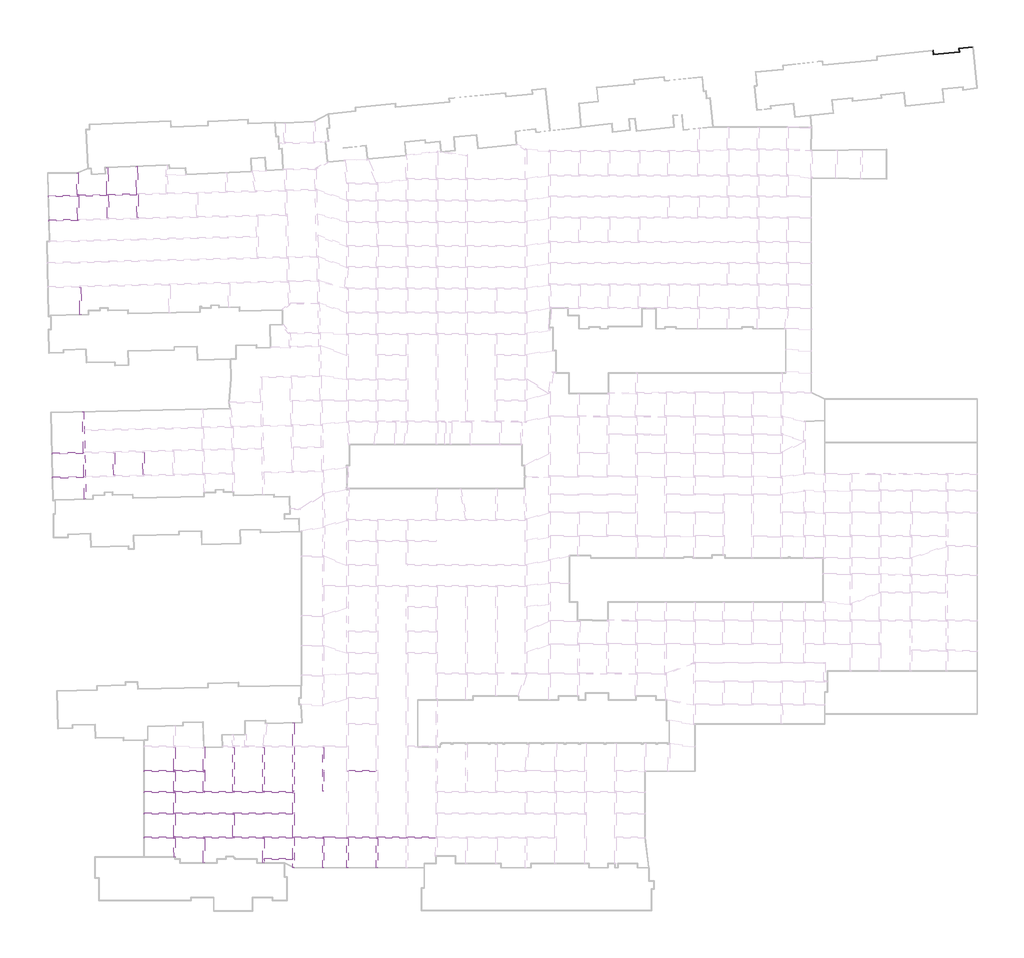
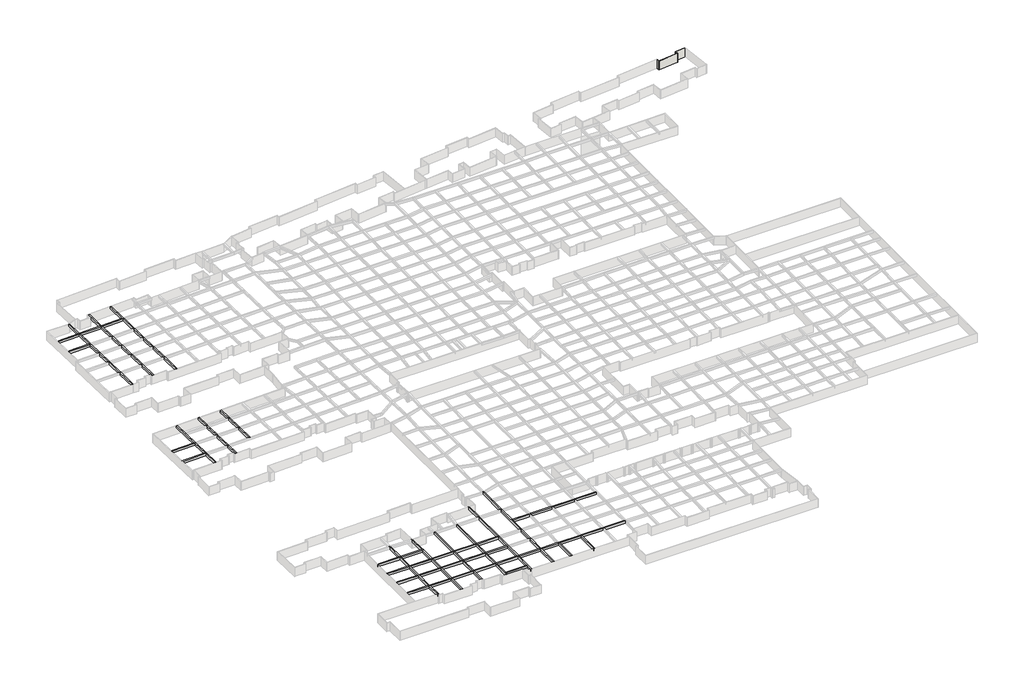
# One storey, part 8 of 20: 42 beams, 4 walls.
"""IFC4 building model written with IfcOpenShell, lengths in millimetres."""

from ifc_helpers import new_model, si_unit, frame, origin, place, context, project, spatial, polyline, outline, extrude, faceted_brep, element, save

model = new_model("IFC4")

# Units and contexts
model_context = context("Model", 3, world=origin())
ifc_project = project(units=[si_unit("LENGTHUNIT", "METRE", prefix="MILLI")], contexts=[model_context])

# Site, building, storey
site = spatial("IfcSite", under=ifc_project)
building = spatial("IfcBuilding", under=site)
storey = spatial("IfcBuildingStorey", under=building, Name="户型图", Elevation=0.0)

# Beams
placement = place(None, origin())
element("IfcBeam", 1, ObjectType="混凝土 - 矩形梁 : KL_beam", at=placement, inside=storey, context=model_context, shape_type="Brep", body=[
    faceted_brep([(-25685.9584576, 180218.1468317, 3300.0), (-25695.523539, 180618.0324519, 3300.0), (-25695.523539, 180618.0324519, 2500.0), (-25685.9584576, 180218.1468317, 2500.0), (-17988.1602694, 180402.2746492, 3300.0), (-17588.2746492, 180411.8397306, 3300.0), (-17597.8397306, 180811.7253508, 3300.0), (-17997.7253508, 180802.1602694, 3300.0), (-17597.8397306, 180811.7253508, 2500.0), (-17997.7253508, 180802.1602694, 2500.0), (-17588.2746492, 180411.8397306, 2500.0), (-17988.1602694, 180402.2746492, 2500.0)], [[[0, 1, 2, 3]], [[1, 0, 4, 5, 6, 7]], [[2, 1, 7, 6, 8, 9]], [[3, 2, 9, 8, 10, 11]], [[0, 3, 11, 10, 5, 4]], [[6, 5, 10, 8]]]),
])
element("IfcBeam", 2, ObjectType="混凝土 - 矩形梁 : KL_beam", at=placement, inside=storey, context=model_context, shape_type="Brep", body=[
    faceted_brep([(-17832.7062646, 173903.2373381, 3300.0), (-17432.8206445, 173912.8024195, 3300.0), (-17442.3866011, 174312.7246305, 3300.0), (-17588.2746492, 180411.8397306, 3300.0), (-17988.1602694, 180402.2746492, 3300.0), (-17842.2713461, 174303.1229582, 3300.0), (-17832.7062646, 173903.2373381, 2500.0), (-17988.1602694, 180402.2746492, 2500.0), (-17842.2713461, 174303.1229582, 2500.0), (-17432.8206445, 173912.8024195, 2500.0), (-17588.2746492, 180411.8397306, 2500.0), (-17442.3866011, 174312.7246305, 2500.0)], [[[0, 1, 2, 3, 4, 5]], [[6, 0, 5, 4, 7, 8]], [[9, 6, 8, 7, 10, 11]], [[1, 9, 11, 10, 3, 2]], [[4, 3, 10, 7]], [[1, 0, 6, 9]]]),
])
element("IfcBeam", 3, ObjectType="混凝土 - 矩形梁 : KL_beam", at=placement, inside=storey, context=model_context, shape_type="SweptSolid", body=[
    extrude(outline(polyline([(-25579.9010779, 173717.9279759), (-25589.4661593, 174117.813596), (-17842.2713461, 174303.1229582), (-17832.7062646, 173903.2373381), (-25579.9010779, 173717.9279759)])), frame((0.0, 0.0, 2500.0), z_axis=(0.0, 0.0, 1.0), x_axis=(1.0, 0.0, 0.0)), (0.0, 0.0, 1.0), 800.0),
])
element("IfcBeam", 4, ObjectType="混凝土 - 矩形梁 : KL_beam", at=placement, inside=storey, context=model_context, shape_type="SweptSolid", body=[
    extrude(outline(polyline([(-17597.8397306, 180811.7253508), (-17997.7253508, 180802.1602694), (-18138.5658972, 186690.2553865), (-17949.102694, 186690.2553865), (-17740.5687803, 186778.7727812), (-17597.8397306, 180811.7253508)])), frame((0.0, 0.0, 2500.0), z_axis=(0.0, 0.0, 1.0), x_axis=(1.0, 0.0, 0.0)), (0.0, 0.0, 1.0), 800.0),
])
element("IfcBeam", 5, ObjectType="混凝土 - 矩形梁 : KL_beam", at=placement, inside=storey, context=model_context, shape_type="SweptSolid", body=[
    extrude(outline(polyline([(-17588.2750768, 180411.8576065), (-17597.8401582, 180811.7432282), (-9999.8837416, 180994.1625895), (-9990.2703339, 180594.278128), (-17588.2750768, 180411.8576065)])), frame((0.0, 0.0, 2500.0), z_axis=(0.0, 0.0, 1.0), x_axis=(1.0, 0.0, 0.0)), (0.0, 0.0, 1.0), 800.0),
])
element("IfcBeam", 6, ObjectType="混凝土 - 矩形梁 : KL_beam", at=placement, inside=storey, context=model_context, shape_type="SweptSolid", body=[
    extrude(outline(polyline([(-9590.3861591, 180603.9034521), (-9599.9995668, 181003.7879151), (-2006.664785, 181187.0229254), (-1996.9546451, 180787.1407967), (-9590.3861591, 180603.9034521)])), frame((0.0, 0.0, 2500.0), z_axis=(0.0, 0.0, 1.0), x_axis=(1.0, 0.0, 0.0)), (0.0, 0.0, 1.0), 800.0),
])
element("IfcBeam", 7, ObjectType="混凝土 - 矩形梁 : KL_beam", at=placement, inside=storey, context=model_context, shape_type="SweptSolid", body=[
    extrude(outline(polyline([(-16823.0159443, 148613.9916157), (-17222.8998075, 148604.3533596), (-17401.6326758, 156019.8431266), (-17001.7470489, 156029.4082082), (-16823.0159443, 148613.9916157)])), frame((0.0, 0.0, 2500.0), z_axis=(0.0, 0.0, 1.0), x_axis=(1.0, 0.0, 0.0)), (0.0, 0.0, 1.0), 800.0),
    extrude(outline(polyline([(-17832.6696806, 173903.2382131), (-17432.7840537, 173912.8032947), (-17306.2945554, 168664.8509217), (-17706.1801823, 168655.2858401), (-17832.6696806, 173903.2382131)])), frame((0.0, 0.0, 2500.0), z_axis=(0.0, 0.0, 1.0), x_axis=(1.0, 0.0, 0.0)), (0.0, 0.0, 1.0), 800.0),
    extrude(outline(polyline([(-17696.541926, 168255.4019703), (-17296.6562991, 168264.9670519), (-17167.7594012, 162917.1335125), (-17567.6433405, 162907.4984183), (-17696.541926, 168255.4019703)])), frame((0.0, 0.0, 2500.0), z_axis=(0.0, 0.0, 1.0), x_axis=(1.0, 0.0, 0.0)), (0.0, 0.0, 1.0), 800.0),
    extrude(outline(polyline([(-17558.0050844, 162507.6145551), (-17158.121145, 162517.2496493), (-17011.3853052, 156429.292078), (-17411.2709321, 156419.7269964), (-17558.0050844, 162507.6145551)])), frame((0.0, 0.0, 2500.0), z_axis=(0.0, 0.0, 1.0), x_axis=(1.0, 0.0, 0.0)), (0.0, 0.0, 1.0), 800.0),
])
element("IfcBeam", 8, ObjectType="混凝土 - 矩形梁 : KL_beam", at=placement, inside=storey, context=model_context, shape_type="Brep", body=[
    faceted_brep([(-8850.0626403, 149809.0093189, 3300.0), (-9249.9471016, 149799.3959113, 3300.0), (-9249.9471016, 149799.3959113, 2500.0), (-8850.0626403, 149809.0093189, 2500.0), (-9004.2027939, 156220.7058147, 3300.0), (-9404.088417, 156211.1407332, 3300.0), (-9404.088417, 156211.1407332, 2500.0), (-9004.2027939, 156220.7058147, 2500.0)], [[[0, 1, 2, 3]], [[1, 0, 4, 5]], [[2, 1, 5, 6]], [[3, 2, 6, 7]], [[0, 3, 7, 4]], [[5, 4, 7, 6]]]),
    faceted_brep([(-10170.4329888, 188088.4205433, 3300.0), (-9770.7457256, 188106.2367096, 3300.0), (-9770.7457256, 188106.2367096, 2500.0), (-10170.4329888, 188088.4205433, 2500.0), (-9443.7780087, 174505.5122009, 3300.0), (-9843.6618727, 174495.8739447, 3300.0), (-9843.6618727, 174495.8739447, 2500.0), (-9443.7780087, 174505.5122009, 2500.0), (-9999.8837416, 180994.1625895, 3300.0), (-9990.2703339, 180594.278128, 3300.0), (-9590.3861591, 180603.9034521, 3300.0), (-9599.9995668, 181003.7879151, 3300.0), (-9999.8837416, 180994.1625895, 2500.0), (-9990.2703339, 180594.278128, 2500.0), (-9599.9995668, 181003.7879151, 2500.0), (-9590.3861591, 180603.9034521, 2500.0)], [[[0, 1, 2, 3]], [[4, 5, 6, 7]], [[1, 0, 8, 9, 5, 4, 10, 11]], [[0, 3, 12, 13, 6, 5, 9, 8]], [[3, 2, 14, 15, 7, 6, 13, 12]], [[2, 1, 11, 10, 4, 7, 15, 14]]]),
    faceted_brep([(-9834.048465, 174095.9894827, 3300.0), (-9434.164601, 174105.6277388, 3300.0), (-9434.164601, 174105.6277388, 2500.0), (-9834.048465, 174095.9894827, 2500.0), (-9307.9651408, 168856.1673089, 3300.0), (-9707.8507639, 168846.6022274, 3300.0), (-9707.8507639, 168846.6022274, 2500.0), (-9307.9651408, 168856.1673089, 2500.0)], [[[0, 1, 2, 3]], [[4, 5, 6, 7]], [[1, 0, 5, 4]], [[0, 3, 6, 5]], [[3, 2, 7, 6]], [[2, 1, 4, 7]]]),
    faceted_brep([(-9698.2373562, 168446.7177632, 3300.0), (-9298.3517331, 168456.2828447, 3300.0), (-9298.3517331, 168456.2828447, 2500.0), (-9698.2373562, 168446.7177632, 2500.0), (-9169.8208105, 163109.841657, 3300.0), (-9569.7047505, 163100.2065627, 3300.0), (-9569.7047505, 163100.2065627, 2500.0), (-9169.8208105, 163109.841657, 2500.0)], [[[0, 1, 2, 3]], [[4, 5, 6, 7]], [[1, 0, 5, 4]], [[0, 3, 6, 5]], [[3, 2, 7, 6]], [[2, 1, 4, 7]]]),
    faceted_brep([(-9560.0913428, 162700.3221009, 3300.0), (-9160.2074028, 162709.9571951, 3300.0), (-9160.2074028, 162709.9571951, 2500.0), (-9560.0913428, 162700.3221009, 2500.0), (-9013.8162016, 156620.5902789, 3300.0), (-9413.7018247, 156611.0251974, 3300.0), (-9413.7018247, 156611.0251974, 2500.0), (-9013.8162016, 156620.5902789, 2500.0)], [[[0, 1, 2, 3]], [[4, 5, 6, 7]], [[1, 0, 5, 4]], [[0, 3, 6, 5]], [[3, 2, 7, 6]], [[2, 1, 4, 7]]]),
])
element("IfcBeam", 9, ObjectType="混凝土 - 矩形梁 : KL_beam", at=placement, inside=storey, context=model_context, shape_type="Brep", body=[
    faceted_brep([(-1224.9412784, 148994.1538412, 3300.0), (-1224.9412784, 148994.1538412, 2500.0), (-825.0591543, 149003.8639809, 2500.0), (-825.0591543, 149003.8639809, 3300.0), (-1404.8339776, 156402.4792466, 3300.0), (-1004.9483311, 156412.0443286, 3300.0), (-1004.9483311, 156412.0443286, 2500.0), (-1404.8339776, 156402.4792466, 2500.0)], [[[0, 1, 2, 3]], [[4, 5, 6, 7]], [[0, 3, 5, 4]], [[3, 2, 6, 5]], [[2, 1, 7, 6]], [[1, 0, 4, 7]]]),
    faceted_brep([(-1783.2084216, 188462.2833149, 3300.0), (-2182.8937132, 188444.4672364, 3300.0), (-2006.664785, 181187.0229254, 3300.0), (-1996.9546451, 180787.1407967, 3300.0), (-1848.8660596, 174688.5696172, 3300.0), (-1448.98219, 174698.2078735, 3300.0), (-1597.0758138, 180796.9865396, 3300.0), (-1606.785957, 181196.8688079, 3300.0), (-1783.2084216, 188462.2833149, 2500.0), (-1448.98219, 174698.2078735, 2500.0), (-1597.0758138, 180796.9865396, 2500.0), (-1606.785957, 181196.8688079, 2500.0), (-2182.8937132, 188444.4672364, 2500.0), (-1848.8660596, 174688.5696172, 2500.0), (-1996.9546451, 180787.1407967, 2500.0), (-2006.664785, 181187.0229254, 2500.0)], [[[0, 1, 2, 3, 4, 5, 6, 7]], [[8, 0, 7, 6, 5, 9, 10, 11]], [[12, 8, 11, 10, 9, 13, 14, 15]], [[1, 12, 15, 14, 13, 4, 3, 2]], [[1, 0, 8, 12]], [[5, 4, 13, 9]]]),
    faceted_brep([(-1839.1559197, 174288.6874866, 3300.0), (-1439.2720501, 174298.3257429, 3300.0), (-1439.2720501, 174298.3257429, 2500.0), (-1839.1559197, 174288.6874866, 2500.0), (-1711.65286, 169037.8676298, 3300.0), (-1311.7672135, 169047.4327119, 3300.0), (-1311.7672135, 169047.4327119, 2500.0), (-1711.65286, 169037.8676298, 2500.0)], [[[0, 1, 2, 3]], [[1, 0, 4, 5]], [[2, 1, 5, 6]], [[3, 2, 6, 7]], [[0, 3, 7, 4]], [[5, 4, 7, 6]]]),
    faceted_brep([(-1701.9427196, 168637.9854794, 3300.0), (-1302.0570732, 168647.5505615, 3300.0), (-1302.0570732, 168647.5505615, 2500.0), (-1701.9427196, 168637.9854794, 2500.0), (-1572.1507865, 163292.9054397, 3300.0), (-1172.2668401, 163302.5405341, 3300.0), (-1172.2668401, 163302.5405341, 2500.0), (-1572.1507865, 163292.9054397, 2500.0)], [[[0, 1, 2, 3]], [[1, 0, 4, 5]], [[2, 1, 5, 6]], [[3, 2, 6, 7]], [[0, 3, 7, 4]], [[5, 4, 7, 6]]]),
    faceted_brep([(-1562.4406466, 162893.0233086, 3300.0), (-1162.5567002, 162902.658403, 3300.0), (-1162.5567002, 162902.658403, 2500.0), (-1562.4406466, 162893.0233086, 2500.0), (-1414.5441179, 156802.361397, 3300.0), (-1014.6584715, 156811.926479, 3300.0), (-1014.6584715, 156811.926479, 2500.0), (-1414.5441179, 156802.361397, 2500.0)], [[[0, 1, 2, 3]], [[1, 0, 4, 5]], [[2, 1, 5, 6]], [[3, 2, 6, 7]], [[0, 3, 7, 4]], [[5, 4, 7, 6]]]),
])
element("IfcBeam", 10, ObjectType="混凝土 - 矩形梁 : KL_beam", at=placement, inside=storey, context=model_context, shape_type="SweptSolid", body=[
    extrude(outline(polyline([(54450.0, 26240.0), (54450.0, 25840.0), (48350.0, 25840.0), (48350.0, 26240.0), (54450.0, 26240.0)])), frame((0.0, 0.0, 2500.0), z_axis=(0.0, 0.0, 1.0), x_axis=(1.0, 0.0, 0.0)), (0.0, 0.0, 1.0), 800.0),
    extrude(outline(polyline([(78450.0, 26240.0), (78450.0, 25840.0), (70850.0, 25840.0), (70850.0, 26240.0), (78450.0, 26240.0)])), frame((0.0, 0.0, 2500.0), z_axis=(0.0, 0.0, 1.0), x_axis=(1.0, 0.0, 0.0)), (0.0, 0.0, 1.0), 800.0),
    extrude(outline(polyline([(70450.0, 26240.0), (70450.0, 25840.0), (62850.0, 25840.0), (62850.0, 26240.0), (70450.0, 26240.0)])), frame((0.0, 0.0, 2500.0), z_axis=(0.0, 0.0, 1.0), x_axis=(1.0, 0.0, 0.0)), (0.0, 0.0, 1.0), 800.0),
    extrude(outline(polyline([(62450.0, 26240.0), (62450.0, 25840.0), (54850.0, 25840.0), (54850.0, 26240.0), (62450.0, 26240.0)])), frame((0.0, 0.0, 2500.0), z_axis=(0.0, 0.0, 1.0), x_axis=(1.0, 0.0, 0.0)), (0.0, 0.0, 1.0), 800.0),
])
element("IfcBeam", 11, ObjectType="混凝土 - 矩形梁 : KL_beam", at=placement, inside=storey, context=model_context, shape_type="Brep", body=[
    faceted_brep([(78450.0, 7940.0, 3300.0), (78450.0, 8340.0, 3300.0), (70850.0, 8340.0, 3300.0), (70450.0, 8340.0, 3300.0), (62850.0, 8340.0, 3300.0), (62450.0, 8340.0, 3300.0), (54850.0, 8340.0, 3300.0), (54450.0, 8340.0, 3300.0), (48350.0, 8340.0, 3300.0), (47950.0, 8340.0, 3300.0), (40351.7306283, 8340.0, 3300.0), (40351.7306283, 7940.0, 3300.0), (47950.0, 7940.0, 3300.0), (48350.0, 7940.0, 3300.0), (54450.0, 7940.0, 3300.0), (54850.0, 7940.0, 3300.0), (62450.0, 7940.0, 3300.0), (62850.0, 7940.0, 3300.0), (70450.0, 7940.0, 3300.0), (70850.0, 7940.0, 3300.0), (78440.7384461, 7940.0, 3300.0), (78450.0, 8340.0, 2500.0), (70850.0, 8340.0, 2500.0), (70450.0, 8340.0, 2500.0), (62850.0, 8340.0, 2500.0), (62450.0, 8340.0, 2500.0), (54850.0, 8340.0, 2500.0), (54450.0, 8340.0, 2500.0), (48350.0, 8340.0, 2500.0), (47950.0, 8340.0, 2500.0), (40351.7306283, 8340.0, 2500.0), (78450.0, 7940.0, 2500.0), (78440.7384461, 7940.0, 2500.0), (70850.0, 7940.0, 2500.0), (70450.0, 7940.0, 2500.0), (62850.0, 7940.0, 2500.0), (62450.0, 7940.0, 2500.0), (54850.0, 7940.0, 2500.0), (54450.0, 7940.0, 2500.0), (48350.0, 7940.0, 2500.0), (47950.0, 7940.0, 2500.0), (40351.7306283, 7940.0, 2500.0)], [[[0, 1, 2, 3, 4, 5, 6, 7, 8, 9, 10, 11, 12, 13, 14, 15, 16, 17, 18, 19, 20]], [[1, 21, 22, 23, 24, 25, 26, 27, 28, 29, 30, 10, 9, 8, 7, 6, 5, 4, 3, 2]], [[21, 31, 32, 33, 34, 35, 36, 37, 38, 39, 40, 41, 30, 29, 28, 27, 26, 25, 24, 23, 22]], [[31, 0, 20, 19, 18, 17, 16, 15, 14, 13, 12, 11, 41, 40, 39, 38, 37, 36, 35, 34, 33, 32]], [[1, 0, 31, 21]], [[11, 10, 30, 41]]]),
])
element("IfcBeam", 12, ObjectType="混凝土 - 矩形梁 : KL_beam", at=placement, inside=storey, context=model_context, shape_type="SweptSolid", body=[
    extrude(outline(polyline([(23892.5739519, 32340.0), (24292.5739519, 32340.0), (24292.5739519, 20540.0), (23892.5739519, 20540.0), (23892.5739519, 32340.0)])), frame((0.0, 0.0, 2500.0), z_axis=(0.0, 0.0, 1.0), x_axis=(1.0, 0.0, 0.0)), (0.0, 0.0, 1.0), 800.0),
])
element("IfcBeam", 13, ObjectType="混凝土 - 矩形梁 : KL_beam", at=placement, inside=storey, context=model_context, shape_type="SweptSolid", body=[
    extrude(outline(polyline([(31950.0, 32340.0), (32350.0, 32340.0), (32350.0, 20540.0), (31950.0, 20540.0), (31950.0, 32340.0)])), frame((0.0, 0.0, 2500.0), z_axis=(0.0, 0.0, 1.0), x_axis=(1.0, 0.0, 0.0)), (0.0, 0.0, 1.0), 800.0),
])
element("IfcBeam", 14, ObjectType="混凝土 - 矩形梁 : KL_beam", at=placement, inside=storey, context=model_context, shape_type="Brep", body=[
    faceted_brep([(40351.7306283, 38946.111756, 3300.0), (40351.7306283, 38946.111756, 2500.0), (39951.7306283, 38946.111756, 2500.0), (39951.7306283, 38946.111756, 3300.0), (39951.7306283, 32740.0, 3300.0), (39951.7306283, 32340.0, 3300.0), (39951.7306283, 20540.0, 3300.0), (40351.7306283, 20540.0, 3300.0), (40351.7306283, 32340.0, 3300.0), (40351.7306283, 32740.0, 3300.0), (39951.7306283, 32740.0, 2500.0), (39951.7306283, 32340.0, 2500.0), (39951.7306283, 20540.0, 2500.0), (40351.7306283, 32740.0, 2500.0), (40351.7306283, 32340.0, 2500.0), (40351.7306283, 20540.0, 2500.0)], [[[0, 1, 2, 3]], [[0, 3, 4, 5, 6, 7, 8, 9]], [[3, 2, 10, 11, 12, 6, 5, 4]], [[2, 1, 13, 14, 15, 12, 11, 10]], [[1, 0, 9, 8, 7, 15, 14, 13]], [[7, 6, 12, 15]]]),
])
element("IfcBeam", 15, ObjectType="混凝土 - 矩形梁 : KL_beam", at=placement, inside=storey, context=model_context, shape_type="Brep", body=[
    faceted_brep([(7945.5604023, 20540.0, 3300.0), (7945.5604023, 20140.0, 3300.0), (8345.5604023, 20140.0, 3300.0), (15956.0, 20140.0, 3300.0), (16356.0, 20140.0, 3300.0), (23892.5739519, 20140.0, 3300.0), (24292.5739519, 20140.0, 3300.0), (31950.0, 20140.0, 3300.0), (32350.0, 20140.0, 3300.0), (39951.7306283, 20140.0, 3300.0), (39951.7306283, 20540.0, 3300.0), (32350.0, 20540.0, 3300.0), (31950.0, 20540.0, 3300.0), (24292.5739519, 20540.0, 3300.0), (23892.5739519, 20540.0, 3300.0), (16356.0, 20540.0, 3300.0), (15956.0, 20540.0, 3300.0), (8345.5604023, 20540.0, 3300.0), (7945.5604023, 20540.0, 2500.0), (39951.7306283, 20540.0, 2500.0), (32350.0, 20540.0, 2500.0), (31950.0, 20540.0, 2500.0), (24292.5739519, 20540.0, 2500.0), (23892.5739519, 20540.0, 2500.0), (16356.0, 20540.0, 2500.0), (15956.0, 20540.0, 2500.0), (8345.5604023, 20540.0, 2500.0), (7945.5604023, 20140.0, 2500.0), (39951.7306283, 20140.0, 2500.0), (32350.0, 20140.0, 2500.0), (31950.0, 20140.0, 2500.0), (24292.5739519, 20140.0, 2500.0), (23892.5739519, 20140.0, 2500.0), (16356.0, 20140.0, 2500.0), (15956.0, 20140.0, 2500.0), (8345.5604023, 20140.0, 2500.0)], [[[0, 1, 2, 3, 4, 5, 6, 7, 8, 9, 10, 11, 12, 13, 14, 15, 16, 17]], [[18, 0, 17, 16, 15, 14, 13, 12, 11, 10, 19, 20, 21, 22, 23, 24, 25, 26]], [[27, 18, 26, 25, 24, 23, 22, 21, 20, 19, 28, 29, 30, 31, 32, 33, 34, 35]], [[1, 27, 35, 34, 33, 32, 31, 30, 29, 28, 9, 8, 7, 6, 5, 4, 3, 2]], [[10, 9, 28, 19]], [[1, 0, 18, 27]]]),
])
element("IfcBeam", 16, ObjectType="混凝土 - 矩形梁 : KL_beam", at=placement, inside=storey, context=model_context, shape_type="Brep", body=[
    faceted_brep([(39951.7306283, 14440.0, 3300.0), (39951.7306283, 14840.0, 3300.0), (32350.0, 14840.0, 3300.0), (31950.0, 14840.0, 3300.0), (24292.5739519, 14840.0, 3300.0), (23892.5739519, 14840.0, 3300.0), (16356.0, 14840.0, 3300.0), (15956.0, 14840.0, 3300.0), (8345.5604023, 14840.0, 3300.0), (8345.5604023, 14440.0, 3300.0), (15956.0, 14440.0, 3300.0), (16356.0, 14440.0, 3300.0), (23892.5739519, 14440.0, 3300.0), (24292.5739519, 14440.0, 3300.0), (31950.0, 14440.0, 3300.0), (32350.0, 14440.0, 3300.0), (39951.7306283, 14440.0, 2500.0), (8345.5604023, 14440.0, 2500.0), (15956.0, 14440.0, 2500.0), (16356.0, 14440.0, 2500.0), (23892.5739519, 14440.0, 2500.0), (24292.5739519, 14440.0, 2500.0), (31950.0, 14440.0, 2500.0), (32350.0, 14440.0, 2500.0), (39951.7306283, 14840.0, 2500.0), (8345.5604023, 14840.0, 2500.0), (15956.0, 14840.0, 2500.0), (16356.0, 14840.0, 2500.0), (23892.5739519, 14840.0, 2500.0), (24292.5739519, 14840.0, 2500.0), (31950.0, 14840.0, 2500.0), (32350.0, 14840.0, 2500.0)], [[[0, 1, 2, 3, 4, 5, 6, 7, 8, 9, 10, 11, 12, 13, 14, 15]], [[16, 0, 15, 14, 13, 12, 11, 10, 9, 17, 18, 19, 20, 21, 22, 23]], [[24, 16, 23, 22, 21, 20, 19, 18, 17, 25, 26, 27, 28, 29, 30, 31]], [[1, 24, 31, 30, 29, 28, 27, 26, 25, 8, 7, 6, 5, 4, 3, 2]], [[1, 0, 16, 24]], [[9, 8, 25, 17]]]),
])
element("IfcBeam", 17, ObjectType="混凝土 - 矩形梁 : KL_beam", at=placement, inside=storey, context=model_context, shape_type="Brep", body=[
    faceted_brep([(7945.5604023, 8340.0, 3300.0), (7945.5604023, 7940.0, 3300.0), (7951.9679234, 7940.0, 3300.0), (8352.1799995, 7940.0, 3300.0), (15956.0, 7940.0, 3300.0), (16356.0, 7940.0, 3300.0), (23892.5739519, 7940.0, 3300.0), (24292.5739519, 7940.0, 3300.0), (31950.0, 7940.0, 3300.0), (32350.0, 7940.0, 3300.0), (39951.7306283, 7940.0, 3300.0), (39951.7306283, 8340.0, 3300.0), (32350.0, 8340.0, 3300.0), (31950.0, 8340.0, 3300.0), (24292.5739519, 8340.0, 3300.0), (23892.5739519, 8340.0, 3300.0), (16356.0, 8340.0, 3300.0), (15956.0, 8340.0, 3300.0), (8345.5604023, 8340.0, 3300.0), (7945.5604023, 8340.0, 2500.0), (39951.7306283, 8340.0, 2500.0), (32350.0, 8340.0, 2500.0), (31950.0, 8340.0, 2500.0), (24292.5739519, 8340.0, 2500.0), (23892.5739519, 8340.0, 2500.0), (16356.0, 8340.0, 2500.0), (15956.0, 8340.0, 2500.0), (8345.5604023, 8340.0, 2500.0), (7945.5604023, 7940.0, 2500.0), (39951.7306283, 7940.0, 2500.0), (32350.0, 7940.0, 2500.0), (31950.0, 7940.0, 2500.0), (24292.5739519, 7940.0, 2500.0), (23892.5739519, 7940.0, 2500.0), (16356.0, 7940.0, 2500.0), (15956.0, 7940.0, 2500.0), (8352.1799995, 7940.0, 2500.0), (7951.9679234, 7940.0, 2500.0)], [[[0, 1, 2, 3, 4, 5, 6, 7, 8, 9, 10, 11, 12, 13, 14, 15, 16, 17, 18]], [[19, 0, 18, 17, 16, 15, 14, 13, 12, 11, 20, 21, 22, 23, 24, 25, 26, 27]], [[28, 19, 27, 26, 25, 24, 23, 22, 21, 20, 29, 30, 31, 32, 33, 34, 35, 36, 37]], [[1, 28, 37, 36, 35, 34, 33, 32, 31, 30, 29, 10, 9, 8, 7, 6, 5, 4, 3, 2]], [[11, 10, 29, 20]], [[1, 0, 19, 28]]]),
])
element("IfcBeam", 18, ObjectType="混凝土 - 矩形梁 : KL_beam", at=placement, inside=storey, context=model_context, shape_type="SweptSolid", body=[
    extrude(outline(polyline([(16356.0, 1311.0), (15956.0, 1311.0), (15956.0, 7940.0), (16356.0, 7940.0), (16356.0, 1311.0)])), frame((0.0, 0.0, 2500.0), z_axis=(0.0, 0.0, 1.0), x_axis=(1.0, 0.0, 0.0)), (0.0, 0.0, 1.0), 800.0),
    extrude(outline(polyline([(15956.0, 20140.0), (16356.0, 20140.0), (16356.0, 14840.0), (15956.0, 14840.0), (15956.0, 20140.0)])), frame((0.0, 0.0, 2500.0), z_axis=(0.0, 0.0, 1.0), x_axis=(1.0, 0.0, 0.0)), (0.0, 0.0, 1.0), 800.0),
    extrude(outline(polyline([(15956.0, 14440.0), (16356.0, 14440.0), (16356.0, 8340.0), (15956.0, 8340.0), (15956.0, 14440.0)])), frame((0.0, 0.0, 2500.0), z_axis=(0.0, 0.0, 1.0), x_axis=(1.0, 0.0, 0.0)), (0.0, 0.0, 1.0), 800.0),
])
element("IfcBeam", 19, ObjectType="混凝土 - 矩形梁 : KL_beam", at=placement, inside=storey, context=model_context, shape_type="SweptSolid", body=[
    extrude(outline(polyline([(24292.5739519, 3040.0), (23892.5739519, 3040.0), (23892.5739519, 7940.0), (24292.5739519, 7940.0), (24292.5739519, 3040.0)])), frame((0.0, 0.0, 2500.0), z_axis=(0.0, 0.0, 1.0), x_axis=(1.0, 0.0, 0.0)), (0.0, 0.0, 1.0), 800.0),
    extrude(outline(polyline([(23892.5739519, 20140.0), (24292.5739519, 20140.0), (24292.5739519, 14840.0), (23892.5739519, 14840.0), (23892.5739519, 20140.0)])), frame((0.0, 0.0, 2500.0), z_axis=(0.0, 0.0, 1.0), x_axis=(1.0, 0.0, 0.0)), (0.0, 0.0, 1.0), 800.0),
    extrude(outline(polyline([(23892.5739519, 14440.0), (24292.5739519, 14440.0), (24292.5739519, 8340.0), (23892.5739519, 8340.0), (23892.5739519, 14440.0)])), frame((0.0, 0.0, 2500.0), z_axis=(0.0, 0.0, 1.0), x_axis=(1.0, 0.0, 0.0)), (0.0, 0.0, 1.0), 800.0),
])
element("IfcBeam", 20, ObjectType="混凝土 - 矩形梁 : KL_beam", at=placement, inside=storey, context=model_context, shape_type="Brep", body=[
    faceted_brep([(32350.0, 1311.0, 3300.0), (31950.0, 1311.0, 3300.0), (31950.0, 1311.0, 2500.0), (32350.0, 1311.0, 2500.0), (32350.0, 2170.0, 3300.0), (32350.0, 2570.0, 3300.0), (32350.0, 7940.0, 3300.0), (31950.0, 7940.0, 3300.0), (31950.0, 7940.0, 2500.0), (32350.0, 7940.0, 2500.0), (32350.0, 2570.0, 2500.0), (32350.0, 2170.0, 2500.0)], [[[0, 1, 2, 3]], [[1, 0, 4, 5, 6, 7]], [[2, 1, 7, 8]], [[3, 2, 8, 9, 10, 11]], [[0, 3, 11, 10, 9, 6, 5, 4]], [[7, 6, 9, 8]]]),
    faceted_brep([(31950.0, 20140.0, 3300.0), (32350.0, 20140.0, 3300.0), (32350.0, 20140.0, 2500.0), (31950.0, 20140.0, 2500.0), (32350.0, 14840.0, 3300.0), (31950.0, 14840.0, 3300.0), (31950.0, 14840.0, 2500.0), (32350.0, 14840.0, 2500.0)], [[[0, 1, 2, 3]], [[4, 5, 6, 7]], [[1, 0, 5, 4]], [[0, 3, 6, 5]], [[3, 2, 7, 6]], [[2, 1, 4, 7]]]),
    faceted_brep([(31950.0, 14440.0, 3300.0), (32350.0, 14440.0, 3300.0), (32350.0, 14440.0, 2500.0), (31950.0, 14440.0, 2500.0), (32350.0, 8340.0, 3300.0), (31950.0, 8340.0, 3300.0), (31950.0, 8340.0, 2500.0), (32350.0, 8340.0, 2500.0)], [[[0, 1, 2, 3]], [[4, 5, 6, 7]], [[1, 0, 5, 4]], [[0, 3, 6, 5]], [[3, 2, 7, 6]], [[2, 1, 4, 7]]]),
])
element("IfcBeam", 21, ObjectType="混凝土 - 矩形梁 : KL_beam", at=placement, inside=storey, context=model_context, shape_type="Brep", body=[
    faceted_brep([(40351.7306283, -3.2601879, 3300.0), (39951.7306283, -3.2601879, 3300.0), (39951.7306283, -3.2601879, 2500.0), (40351.7306283, -3.2601879, 2500.0), (40351.7306283, 7940.0, 3300.0), (40351.7306283, 8340.0, 3300.0), (40351.7306283, 14440.0, 3300.0), (40351.7306283, 14840.0, 3300.0), (40351.7306283, 20140.0, 3300.0), (39951.7306283, 20140.0, 3300.0), (39951.7306283, 14840.0, 3300.0), (39951.7306283, 14440.0, 3300.0), (39951.7306283, 8340.0, 3300.0), (39951.7306283, 7940.0, 3300.0), (39951.7306283, 2570.0, 3300.0), (39951.7306283, 2170.0, 3300.0), (39951.7306283, 20140.0, 2500.0), (39951.7306283, 14840.0, 2500.0), (39951.7306283, 14440.0, 2500.0), (39951.7306283, 8340.0, 2500.0), (39951.7306283, 7940.0, 2500.0), (39951.7306283, 2570.0, 2500.0), (39951.7306283, 2170.0, 2500.0), (40351.7306283, 20140.0, 2500.0), (40351.7306283, 14840.0, 2500.0), (40351.7306283, 14440.0, 2500.0), (40351.7306283, 8340.0, 2500.0), (40351.7306283, 7940.0, 2500.0)], [[[0, 1, 2, 3]], [[1, 0, 4, 5, 6, 7, 8, 9, 10, 11, 12, 13, 14, 15]], [[2, 1, 15, 14, 13, 12, 11, 10, 9, 16, 17, 18, 19, 20, 21, 22]], [[3, 2, 22, 21, 20, 19, 18, 17, 16, 23, 24, 25, 26, 27]], [[0, 3, 27, 26, 25, 24, 23, 8, 7, 6, 5, 4]], [[9, 8, 23, 16]]]),
])
element("IfcBeam", 22, ObjectType="混凝土 - 矩形梁 : KL_beam", at=placement, inside=storey, context=model_context, shape_type="SweptSolid", body=[
    extrude(outline(polyline([(32350.0, 2170.0), (32350.0, 2570.0), (39951.7306283, 2570.0), (39951.7306283, 2170.0), (32350.0, 2170.0)])), frame((0.0, 0.0, 2500.0), z_axis=(0.0, 0.0, 1.0), x_axis=(1.0, 0.0, 0.0)), (0.0, 0.0, 1.0), 800.0),
])
element("IfcBeam", 23, ObjectType="混凝土 - 矩形梁 : KL_beam", at=placement, inside=storey, context=model_context, shape_type="Brep", body=[
    faceted_brep([(47950.0, 8340.0, 3300.0), (48350.0, 8340.0, 3300.0), (48350.0, 14440.0, 3300.0), (47950.0, 14440.0, 3300.0), (47950.0, 8340.0, 2500.0), (47950.0, 14440.0, 2500.0), (48350.0, 8340.0, 2500.0), (48350.0, 14440.0, 2500.0)], [[[0, 1, 2, 3]], [[4, 0, 3, 5]], [[6, 4, 5, 7]], [[1, 6, 7, 2]], [[1, 0, 4, 6]], [[3, 2, 7, 5]]]),
    faceted_brep([(48350.0, 14840.0, 3300.0), (47950.0, 14840.0, 3300.0), (47950.0, 14840.0, 2500.0), (48350.0, 14840.0, 2500.0), (48350.0, 20140.0, 3300.0), (47950.0, 20140.0, 3300.0), (47950.0, 20140.0, 2500.0), (48350.0, 20140.0, 2500.0)], [[[0, 1, 2, 3]], [[1, 0, 4, 5]], [[2, 1, 5, 6]], [[3, 2, 6, 7]], [[0, 3, 7, 4]], [[5, 4, 7, 6]]]),
    faceted_brep([(48350.0, 20540.0, 3300.0), (47950.0, 20540.0, 3300.0), (47950.0, 20540.0, 2500.0), (48350.0, 20540.0, 2500.0), (48350.0, 25840.0, 3300.0), (48350.0, 26240.0, 3300.0), (48350.0, 32340.0, 3300.0), (47950.0, 32340.0, 3300.0), (47950.0, 32340.0, 2500.0), (48350.0, 32340.0, 2500.0), (48350.0, 26240.0, 2500.0), (48350.0, 25840.0, 2500.0)], [[[0, 1, 2, 3]], [[1, 0, 4, 5, 6, 7]], [[2, 1, 7, 8]], [[3, 2, 8, 9, 10, 11]], [[0, 3, 11, 10, 9, 6, 5, 4]], [[7, 6, 9, 8]]]),
    faceted_brep([(48350.0, 32740.0, 3300.0), (47950.0, 32740.0, 3300.0), (47950.0, 32740.0, 2500.0), (48350.0, 32740.0, 2500.0), (48350.0, 43852.7641216, 3300.0), (47950.0, 43867.507495, 3300.0), (47950.0, 43467.2358784, 3300.0), (48350.0, 38390.0, 3300.0), (48350.0, 38790.0, 3300.0), (48350.0, 43510.0922713, 3300.0), (47950.0, 43867.507495, 2500.0), (47950.0, 43467.2358784, 2500.0), (48350.0, 43852.7641216, 2500.0), (48350.0, 43510.0922713, 2500.0), (48350.0, 38790.0, 2500.0), (48350.0, 38390.0, 2500.0)], [[[0, 1, 2, 3]], [[4, 5, 6, 1, 0, 7, 8, 9]], [[5, 10, 11, 2, 1, 6]], [[10, 12, 13, 14, 15, 3, 2, 11]], [[12, 4, 9, 8, 7, 0, 3, 15, 14, 13]], [[5, 4, 12, 10]]]),
])
element("IfcBeam", 24, ObjectType="混凝土 - 矩形梁 : KL_beam", at=placement, inside=storey, context=model_context, shape_type="Brep", body=[
    faceted_brep([(16346.5394526, 25840.0, 3300.0), (16346.5394526, 26240.0, 3300.0), (15946.4785214, 26240.0, 3300.0), (8345.5604023, 26240.0, 3300.0), (7945.5604023, 26240.0, 3300.0), (7945.5604023, 25840.0, 3300.0), (8345.5604023, 25840.0, 3300.0), (15956.0, 25840.0, 3300.0), (16346.5394526, 25840.0, 2500.0), (7945.5604023, 25840.0, 2500.0), (8345.5604023, 25840.0, 2500.0), (15956.0, 25840.0, 2500.0), (16346.5394526, 26240.0, 2500.0), (7945.5604023, 26240.0, 2500.0), (8345.5604023, 26240.0, 2500.0), (15946.4785214, 26240.0, 2500.0)], [[[0, 1, 2, 3, 4, 5, 6, 7]], [[8, 0, 7, 6, 5, 9, 10, 11]], [[12, 8, 11, 10, 9, 13, 14, 15]], [[1, 12, 15, 14, 13, 4, 3, 2]], [[1, 0, 8, 12]], [[5, 4, 13, 9]]]),
])
element("IfcBeam", 25, ObjectType="混凝土 - 矩形梁 : KL_beam", at=placement, inside=storey, context=model_context, shape_type="Brep", body=[
    faceted_brep([(16237.4051317, 32492.3010599, 3300.0), (15837.1001969, 32506.2800163, 3300.0), (15844.0907397, 32105.7920834, 3300.0), (15946.4785214, 26240.0, 3300.0), (16346.5394526, 26240.0, 3300.0), (16353.5214786, 25840.0, 3300.0), (16353.5214786, 25840.0, 2500.0), (16350.0304656, 26040.0, 2500.0), (16346.5394526, 26240.0, 2500.0), (16237.4051317, 32492.3010599, 2500.0), (16350.0304656, 26040.0, 3300.0), (15837.1001969, 32506.2800163, 2500.0), (15946.4785214, 26240.0, 2500.0), (15844.0907397, 32105.7920834, 2500.0), (16346.5394526, 25840.0, 3300.0), (16346.5394526, 25840.0, 2500.0)], [[[0, 1, 2, 3, 4]], [[5, 6, 7, 8, 9, 0, 4, 10]], [[11, 9, 8, 12, 13]], [[1, 11, 13, 12, 3, 2]], [[6, 5, 14, 15]], [[8, 4, 3, 12]], [[4, 8, 15, 14]], [[14, 5, 10, 4]], [[8, 7, 6, 15]], [[1, 0, 9, 11]]]),
])
element("IfcBeam", 26, ObjectType="混凝土 - 矩形梁 : KL_beam", at=placement, inside=storey, context=model_context, shape_type="Brep", body=[
    faceted_brep([(7945.5604023, 26240.0, 3300.0), (8345.5604023, 26240.0, 3300.0), (8345.5604023, 32367.6465329, 3300.0), (7945.5604023, 32381.6148407, 3300.0), (7945.5604023, 32374.7525956, 3300.0), (7945.5604023, 32781.8586584, 3300.0), (7945.5604023, 32781.8586584, 2500.0), (7945.5604023, 32774.7525956, 2500.0), (7945.5604023, 32381.6148407, 2500.0), (7945.5604023, 32374.7525956, 2500.0), (7945.5604023, 26240.0, 2500.0), (7945.5604023, 32774.7525956, 3300.0), (8345.5604023, 26240.0, 2500.0), (8345.5604023, 32367.6465329, 2500.0), (7959.5202009, 32781.3711715, 3300.0), (7959.5202009, 32781.3711715, 2500.0)], [[[0, 1, 2, 3, 4]], [[5, 6, 7, 8, 9, 10, 0, 4, 3, 11]], [[12, 10, 9, 8, 13]], [[1, 12, 13, 2]], [[6, 5, 14, 15]], [[1, 0, 10, 12]], [[8, 3, 2, 13]], [[3, 8, 15, 14]], [[14, 5, 11, 3]], [[6, 15, 8, 7]]]),
])
element("IfcBeam", 27, ObjectType="混凝土 - 矩形梁 : KL_beam", at=placement, inside=storey, context=model_context, shape_type="SweptSolid", body=[
    extrude(outline(polyline([(8345.5604023, 20540.0), (7945.5604023, 20540.0), (7945.5604023, 25840.0), (8345.5604023, 25840.0), (8345.5604023, 20540.0)])), frame((0.0, 0.0, 2500.0), z_axis=(0.0, 0.0, 1.0), x_axis=(1.0, 0.0, 0.0)), (0.0, 0.0, 1.0), 800.0),
])
element("IfcBeam", 28, ObjectType="混凝土 - 矩形梁 : KL_beam", at=placement, inside=storey, context=model_context, shape_type="Brep", body=[
    faceted_brep([(16356.0, 26040.0, 3300.0), (16356.0, 26040.0, 2500.0), (16350.0304656, 26040.0, 2500.0), (16350.0304656, 26040.0, 3300.0), (16356.0, 20540.0, 3300.0), (16353.5214786, 25840.0, 3300.0), (16346.5394526, 25840.0, 3300.0), (15956.0, 25840.0, 3300.0), (15956.0, 20540.0, 3300.0), (16356.0, 20540.0, 2500.0), (15956.0, 20540.0, 2500.0), (15956.0, 25840.0, 2500.0), (16346.5394526, 25840.0, 2500.0), (16353.5214786, 25840.0, 2500.0)], [[[0, 1, 2, 3]], [[4, 0, 3, 5, 6, 7, 8]], [[1, 0, 4, 9]], [[1, 9, 10, 11, 12, 13, 2]], [[10, 8, 7, 11]], [[4, 8, 10, 9]], [[5, 13, 12, 11, 7, 6]], [[13, 5, 3, 2]]]),
])
element("IfcBeam", 29, ObjectType="混凝土 - 矩形梁 : KL_beam", at=placement, inside=storey, context=model_context, shape_type="Brep", body=[
    faceted_brep([(8345.5604023, 20140.0, 3300.0), (7945.5604023, 20140.0, 3300.0), (7945.5604023, 14840.0, 3300.0), (7945.5604023, 14440.0, 3300.0), (7945.5604023, 8340.0, 3300.0), (8345.5604023, 8340.0, 3300.0), (8345.5604023, 14440.0, 3300.0), (8345.5604023, 14840.0, 3300.0), (7945.5604023, 20140.0, 2500.0), (7945.5604023, 14840.0, 2500.0), (7945.5604023, 14440.0, 2500.0), (7945.5604023, 8340.0, 2500.0), (8345.5604023, 20140.0, 2500.0), (8345.5604023, 14840.0, 2500.0), (8345.5604023, 14440.0, 2500.0), (8345.5604023, 8340.0, 2500.0)], [[[0, 1, 2, 3, 4, 5, 6, 7]], [[1, 8, 9, 10, 11, 4, 3, 2]], [[8, 12, 13, 14, 15, 11, 10, 9]], [[12, 0, 7, 6, 5, 15, 14, 13]], [[1, 0, 12, 8]], [[5, 4, 11, 15]]]),
])
element("IfcBeam", 30, ObjectType="混凝土 - 矩形梁 : KL_beam", at=placement, inside=storey, context=model_context, shape_type="SweptSolid", body=[
    extrude(outline(polyline([(20.4770061, 7940.0), (20.4770061, 8340.0), (7945.5604023, 8340.0), (7945.5604023, 7940.0), (20.4770061, 7940.0)])), frame((0.0, 0.0, 2500.0), z_axis=(0.0, 0.0, 1.0), x_axis=(1.0, 0.0, 0.0)), (0.0, 0.0, 1.0), 800.0),
])
element("IfcBeam", 31, ObjectType="混凝土 - 矩形梁 : KL_beam", at=placement, inside=storey, context=model_context, shape_type="SweptSolid", body=[
    extrude(outline(polyline([(20.4770061, 14440.0), (20.4770061, 14840.0), (7945.5604023, 14840.0), (7945.5604023, 14440.0), (20.4770061, 14440.0)])), frame((0.0, 0.0, 2500.0), z_axis=(0.0, 0.0, 1.0), x_axis=(1.0, 0.0, 0.0)), (0.0, 0.0, 1.0), 800.0),
])
element("IfcBeam", 32, ObjectType="混凝土 - 矩形梁 : KL_beam", at=placement, inside=storey, context=model_context, shape_type="SweptSolid", body=[
    extrude(outline(polyline([(20.4770061, 20140.0), (20.4770061, 20540.0), (7945.5604023, 20540.0), (7945.5604023, 20140.0), (20.4770061, 20140.0)])), frame((0.0, 0.0, 2500.0), z_axis=(0.0, 0.0, 1.0), x_axis=(1.0, 0.0, 0.0)), (0.0, 0.0, 1.0), 800.0),
])
element("IfcBeam", 33, ObjectType="混凝土 - 矩形梁 : KL_beam", at=placement, inside=storey, context=model_context, shape_type="SweptSolid", body=[
    extrude(outline(polyline([(20.4770061, 25840.0), (20.4770061, 26240.0), (7945.5604023, 26240.0), (7945.5604023, 25840.0), (20.4770061, 25840.0)])), frame((0.0, 0.0, 2500.0), z_axis=(0.0, 0.0, 1.0), x_axis=(1.0, 0.0, 0.0)), (0.0, 0.0, 1.0), 800.0),
])
element("IfcBeam", 34, ObjectType="混凝土 - 矩形梁 : KL_beam", at=placement, inside=storey, context=model_context, shape_type="Brep", body=[
    faceted_brep([(8516.8797857, 2882.8635999, 3300.0), (8117.0917494, 2869.8433848, 3300.0), (8117.0917494, 2869.8433848, 2500.0), (8516.8797857, 2882.8635999, 2500.0), (8352.1799995, 7940.0, 3300.0), (8345.5604023, 7940.0, 3300.0), (7951.9679234, 7940.0, 3300.0), (7951.9679234, 7940.0, 2500.0), (8345.5604023, 7940.0, 2500.0), (8352.1799995, 7940.0, 2500.0)], [[[0, 1, 2, 3]], [[1, 0, 4, 5, 6]], [[2, 1, 6, 7]], [[3, 2, 7, 8, 9]], [[0, 3, 9, 4]], [[7, 6, 5, 4, 9, 8]]]),
])
element("IfcBeam", 35, ObjectType="混凝土 - 矩形梁 : KL_beam", at=placement, inside=storey, context=model_context, shape_type="SweptSolid", body=[
    extrude(outline(polyline([(-24721.2795081, 111118.7813849), (-24730.9207359, 111518.6651764), (-16333.9623528, 111721.1164636), (-16324.3152742, 111321.2328132), (-24721.2795081, 111118.7813849)])), frame((0.0, 0.0, 2500.0), z_axis=(0.0, 0.0, 1.0), x_axis=(1.0, 0.0, 0.0)), (0.0, 0.0, 1.0), 800.0),
])
element("IfcBeam", 36, ObjectType="混凝土 - 矩形梁 : KL_beam", at=placement, inside=storey, context=model_context, shape_type="SweptSolid", body=[
    extrude(outline(polyline([(-24613.4729092, 104619.5953283), (-24623.114137, 105019.4791198), (-16177.1998237, 105223.1107382), (-16167.552745, 104823.2270877), (-24613.4729092, 104619.5953283)])), frame((0.0, 0.0, 2500.0), z_axis=(0.0, 0.0, 1.0), x_axis=(1.0, 0.0, 0.0)), (0.0, 0.0, 1.0), 800.0),
])
element("IfcBeam", 37, ObjectType="混凝土 - 矩形梁 : KL_beam", at=placement, inside=storey, context=model_context, shape_type="Brep", body=[
    faceted_brep([(-16593.9490761, 122497.8959986, 3300.0), (-16194.0654257, 122507.5430772, 3300.0), (-16194.0654257, 122507.5430772, 2500.0), (-16593.9490761, 122497.8959986, 2500.0), (-16333.9623528, 111721.1164636, 3300.0), (-16324.3152742, 111321.2328132, 3300.0), (-16177.1998237, 105223.1107382, 3300.0), (-16167.552745, 104823.2270877, 3300.0), (-16029.3958545, 99096.4486915, 3300.0), (-15629.5122041, 99106.0957701, 3300.0), (-15629.5122041, 99106.0957701, 2500.0), (-16029.3958545, 99096.4486915, 2500.0), (-16167.552745, 104823.2270877, 2500.0), (-16177.1998237, 105223.1107382, 2500.0), (-16324.3152742, 111321.2328132, 2500.0), (-16333.9623528, 111721.1164636, 2500.0)], [[[0, 1, 2, 3]], [[1, 0, 4, 5, 6, 7, 8, 9]], [[2, 1, 9, 10]], [[3, 2, 10, 11, 12, 13, 14, 15]], [[0, 3, 15, 14, 13, 12, 11, 8, 7, 6, 5, 4]], [[9, 8, 11, 10]]]),
])
element("IfcBeam", 38, ObjectType="混凝土 - 矩形梁 : KL_beam", at=placement, inside=storey, context=model_context, shape_type="SweptSolid", body=[
    extrude(outline(polyline([(-8594.9385117, 122691.03911), (-8195.0548612, 122700.6861887), (-8079.7847303, 117922.5930146), (-8479.6685551, 117912.9531635), (-8594.9385117, 122691.03911)])), frame((0.0, 0.0, 2500.0), z_axis=(0.0, 0.0, 1.0), x_axis=(1.0, 0.0, 0.0)), (0.0, 0.0, 1.0), 800.0),
    extrude(outline(polyline([(-7654.6222007, 100299.0667415), (-8054.5058512, 100289.4196628), (-8168.5347415, 105016.0618413), (-7768.6509225, 105025.7019334), (-7654.6222007, 100299.0667415)])), frame((0.0, 0.0, 2500.0), z_axis=(0.0, 0.0, 1.0), x_axis=(1.0, 0.0, 0.0)), (0.0, 0.0, 1.0), 800.0),
    extrude(outline(polyline([(-8470.0214764, 117513.069513), (-8070.1376517, 117522.7093641), (-7935.0605304, 111923.5913086), (-8334.9443493, 111913.9512165), (-8470.0214764, 117513.069513)])), frame((0.0, 0.0, 2500.0), z_axis=(0.0, 0.0, 1.0), x_axis=(1.0, 0.0, 0.0)), (0.0, 0.0, 1.0), 800.0),
    extrude(outline(polyline([(-8325.2972707, 111514.0675661), (-7925.4134517, 111523.7076581), (-7778.2980012, 105425.5855838), (-8178.1818202, 105415.9454918), (-8325.2972707, 111514.0675661)])), frame((0.0, 0.0, 2500.0), z_axis=(0.0, 0.0, 1.0), x_axis=(1.0, 0.0, 0.0)), (0.0, 0.0, 1.0), 800.0),
])
element("IfcBeam", 39, ObjectType="混凝土 - 矩形梁 : KL_beam", at=placement, inside=storey, context=model_context, shape_type="SweptSolid", body=[
    extrude(outline(polyline([(-635.4218685, 122883.0400563), (-235.538077, 122892.6812841), (-120.335014, 118114.4685185), (-520.2188388, 118104.8286674), (-635.4218685, 122883.0400563)])), frame((0.0, 0.0, 2500.0), z_axis=(0.0, 0.0, 1.0), x_axis=(1.0, 0.0, 0.0)), (0.0, 0.0, 1.0), 800.0),
    extrude(outline(polyline([(180.9687495, 105617.4614753), (-218.9150694, 105607.8213832), (-365.9412952, 111705.9456085), (33.9425237, 111715.5857005), (180.9687495, 105617.4614753)])), frame((0.0, 0.0, 2500.0), z_axis=(0.0, 0.0, 1.0), x_axis=(1.0, 0.0, 0.0)), (0.0, 0.0, 1.0), 800.0),
    extrude(outline(polyline([(-510.577611, 117704.9448759), (-110.6937863, 117714.584727), (24.3012959, 112115.4694921), (-375.582523, 112105.8294), (-510.577611, 117704.9448759)])), frame((0.0, 0.0, 2500.0), z_axis=(0.0, 0.0, 1.0), x_axis=(1.0, 0.0, 0.0)), (0.0, 0.0, 1.0), 800.0),
])
element("IfcBeam", 40, ObjectType="混凝土 - 矩形梁 : KL_beam", at=placement, inside=storey, context=model_context, shape_type="SweptSolid", body=[
    extrude(outline(polyline([(48350.0, -3.2601879), (47950.0, -3.2601879), (47950.0, 7940.0), (48350.0, 7940.0), (48350.0, -3.2601879)])), frame((0.0, 0.0, 2500.0), z_axis=(0.0, 0.0, 1.0), x_axis=(1.0, 0.0, 0.0)), (0.0, 0.0, 1.0), 800.0),
])
element("IfcBeam", 41, ObjectType="混凝土 - 矩形梁 : KL_beam", at=placement, inside=storey, context=model_context, shape_type="SweptSolid", body=[
    extrude(outline(polyline([(54850.0, 0.0), (54450.0, 0.0), (54450.0, 7940.0), (54850.0, 7940.0), (54850.0, 0.0)])), frame((0.0, 0.0, 2500.0), z_axis=(0.0, 0.0, 1.0), x_axis=(1.0, 0.0, 0.0)), (0.0, 0.0, 1.0), 800.0),
])
element("IfcBeam", 42, ObjectType="混凝土 - 矩形梁 : KL_beam", at=placement, inside=storey, context=model_context, shape_type="SweptSolid", body=[
    extrude(outline(polyline([(62850.0, 0.0), (62450.0, 0.0), (62450.0, 7940.0), (62850.0, 7940.0), (62850.0, 0.0)])), frame((0.0, 0.0, 2500.0), z_axis=(0.0, 0.0, 1.0), x_axis=(1.0, 0.0, 0.0)), (0.0, 0.0, 1.0), 800.0),
])

# Walls
element("IfcWall", 43, ObjectType="所有墙体", at=placement, inside=storey, context=model_context, shape_type="Brep", body=[
    faceted_brep([(222651.7827909, 220675.7631937, 0.0), (218873.6544292, 220278.6659015, 0.0), (218873.6544292, 220278.6659015, 3300.0), (222651.7827909, 220675.7631937, 3300.0), (222664.3262065, 220556.4205662, 0.0), (222664.3262065, 220556.4205662, 3300.0), (219011.9587337, 220172.5412761, 3300.0), (218892.4523269, 220159.9806466, 3300.0), (218892.4523269, 220159.9806466, 0.0), (219011.9587337, 220172.5412761, 0.0)], [[[0, 1, 2, 3]], [[4, 5, 6, 7, 8, 9]], [[1, 0, 4, 9, 8]], [[3, 2, 7, 6, 5]], [[0, 3, 5, 4]], [[2, 1, 8, 7]]]),
])
element("IfcWall", 44, ObjectType="所有墙体", at=placement, inside=storey, context=model_context, shape_type="Brep", body=[
    faceted_brep([(218892.4523269, 220159.9806466, 0.0), (219030.0888942, 219290.9775609, 0.0), (219048.8867919, 219172.292306, 0.0), (219048.8867919, 219172.292306, 3300.0), (219030.0888942, 219290.9775609, 3300.0), (218892.4523269, 220159.9806466, 3300.0), (219011.9587337, 220172.5412761, 0.0), (219011.9587337, 220172.5412761, 3300.0), (219168.3931987, 219184.8529355, 3300.0), (219168.3931987, 219184.8529355, 0.0)], [[[0, 1, 2, 3, 4, 5]], [[6, 7, 8, 9]], [[2, 1, 0, 6, 9]], [[5, 4, 3, 8, 7]], [[0, 5, 7, 6]], [[3, 2, 9, 8]]]),
])
element("IfcWall", 45, ObjectType="所有墙体", at=placement, inside=storey, context=model_context, shape_type="Brep", body=[
    faceted_brep([(219030.0888942, 219290.9775609, 0.0), (212187.9420335, 218571.8389475, 0.0), (212068.4356267, 218559.278318, 0.0), (212068.4356267, 218559.278318, 3300.0), (212187.9420335, 218571.8389475, 3300.0), (219030.0888942, 219290.9775609, 3300.0), (219048.8867919, 219172.292306, 0.0), (219048.8867919, 219172.292306, 3300.0), (212087.2335243, 218440.5930631, 3300.0), (212087.2335243, 218440.5930631, 0.0)], [[[0, 1, 2, 3, 4, 5]], [[6, 7, 8, 9]], [[2, 1, 0, 6, 9]], [[5, 4, 3, 8, 7]], [[0, 5, 7, 6]], [[3, 2, 9, 8]]]),
])
element("IfcWall", 46, ObjectType="所有墙体", at=placement, inside=storey, context=model_context, shape_type="Brep", body=[
    faceted_brep([(212187.9420335, 218571.8389475, 0.0), (212015.8641219, 219658.2961221, 0.0), (212015.8641219, 219658.2961221, 3300.0), (212187.9420335, 218571.8389475, 3300.0), (212068.4356267, 218559.278318, 0.0), (212068.4356267, 218559.278318, 3300.0), (211915.1556128, 219527.0502378, 3300.0), (211896.3577151, 219645.7354926, 3300.0), (211896.3577151, 219645.7354926, 0.0), (211915.1556128, 219527.0502378, 0.0)], [[[0, 1, 2, 3]], [[4, 5, 6, 7, 8, 9]], [[1, 0, 4, 9, 8]], [[3, 2, 7, 6, 5]], [[0, 3, 5, 4]], [[2, 1, 8, 7]]]),
])

save(model, "model.ifc")

# Revit data of these elements
# Type "混凝土 - 矩形梁 : KL_beam"
#   Length [instance default] = 1524 mm
#   b = 400 mm
#   h = 800 mm
#   Structural Material [instance default] = 混凝土 - 现场浇注混凝土
#   Assembly Code = ""
# Type "所有墙体"
#   Layers, outside or top first: 120 mm "默认" (function 1)
# Elements 1, 2, 3, 4, 5, 6, 7, 8, 9, 10, 11, 12, 13, 14, 15, 16, 17, 18, 19, 20, 21, 22, 23, 24, 25, 26, 27, 28, 29, 30, 31, 32, 33, 34, 35, 36, 37, 38, 39, 40, 41, 42 (IfcBeam, "混凝土 - 矩形梁 : KL_beam")
#   Comments = ""
#   Structural Material = none
#   Phase Created = 新构造
# Elements 43, 44, 45, 46 (IfcWall, "所有墙体")
#   Comments = ""
#   Top Offset = 0 mm
#   Base Offset = 0 mm
#   wall height = 3300 mm
#   Phase Created = 新构造
#   Base Constraint = 户型图
#   Top Constraint = 层高
#   Materials on its faces: "默认"
# Materials
#   "混凝土 - 现场浇注混凝土": class "混凝土", colour RGB 192 192 192, transparency 0
#   "默认": class "其他", colour RGB 192 192 192, transparency 0, Cost = 0
